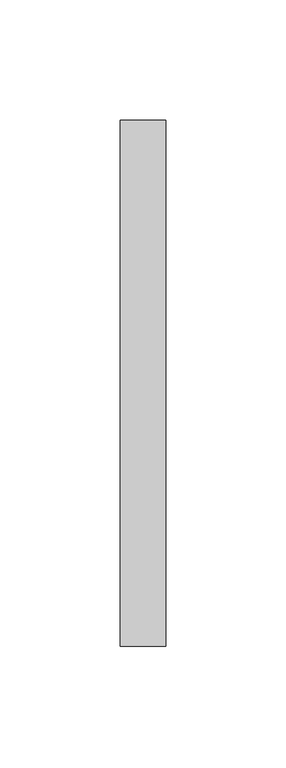
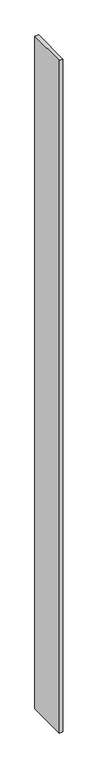
"""IFC4 building model written with IfcOpenShell, lengths in millimetres: proxy geometry, Inner panel1:Inner panel:306176:Inner panel:306176 : Inner panel1:Inner panel:306176:300391:Inner panel:306176:Inner panel:306176 : Inner panel1:Inner panel:306176:300391 : Inner panel1:Inner panel:306176:Inner panel:306176 : Inner panel1:Inner panel:306176:300391:2 : Inner panel1:Inner panel:306176:Inner panel:306176 : Inner panel1:Inner panel:306176:300391:Inner panel:306176:Inner panel:306176 : Inner panel1:Inner panel:306176:300391 : Inner panel1:Inner panel:306176:Inner panel:306176 : Inner panel1:Inner panel:306176:300391:300168."""

from ifc_helpers import new_model, si_unit, frame, origin, place, context, project, spatial, polyline, outline, extrude, source, transform, mapped, element, save


def generic_models_e7d118f8(model_context):
    return source(origin(), model_context, "Body", "SweptSolid", [
        extrude(outline(polyline([(570452.6367239, -578997.5163841), (570433.5867239, -578997.5163841), (570433.5867239, -578778.4413841), (570452.6367239, -578778.4413841), (570452.6367239, -578997.5163841)])), frame((0.0, 0.0, 25.4), z_axis=(0.0, 0.0, 1.0), x_axis=(1.0, 0.0, 0.0)), (0.0, 0.0, 1.0), 3689.35),
    ])


if __name__ == "__main__":
    model = new_model("IFC4")
    model_context = context("Model", 3, world=origin())
    ifc_project = project(units=[si_unit("LENGTHUNIT", "METRE", prefix="MILLI")], contexts=[model_context])
    site = spatial("IfcSite", under=ifc_project)
    building = spatial("IfcBuilding", under=site)
    placement = place(None, origin())
    generic_models_shape = generic_models_e7d118f8(model_context)
    element("IfcBuildingElementProxy", 1, Name="Inner panel1:Inner panel:306176:Inner panel:306176 : Inner panel1:Inner panel:306176:300391:Inner panel:306176:Inner panel:306176 : Inner panel1:Inner panel:306176:300391 : Inner panel1:Inner panel:306176:Inner panel:306176 : Inner panel1:Inner panel:306176:300391:2 : Inner panel1:Inner panel:306176:Inner panel:306176 : Inner panel1:Inner panel:306176:300391:Inner panel:306176:Inner panel:306176 : Inner panel1:Inner panel:306176:300391 : Inner panel1:Inner panel:306176:Inner panel:306176 : Inner panel1:Inner panel:306176:300391:300168", ObjectType="Inner panel1:Inner panel:306176:Inner panel:306176 : Inner panel1:Inner panel:306176:300391:Inner panel:306176:Inner panel:306176 : Inner panel1:Inner panel:306176:300391 : Inner panel1:Inner panel:306176:Inner panel:306176 : Inner panel1:Inner panel:306176:300391:2 : Inner panel1:Inner panel:306176:Inner panel:306176 : Inner panel1:Inner panel:306176:300391:Inner panel:306176:Inner panel:306176 : Inner panel1:Inner panel:306176:300391 : Inner panel1:Inner panel:306176:Inner panel:306176 : Inner panel1:Inner panel:306176:300391:300168", at=placement, inside=building, context=model_context, shape_type="MappedRepresentation", body=[
        mapped(generic_models_shape, transform((0.0, 0.0, 0.0), x_axis=(1.0, 0.0, 0.0), y_axis=(0.0, 1.0, 0.0), z_axis=(0.0, 0.0, 1.0))),
    ])
    save(model, "model.ifc")

# Revit data of these elements
# Type "Inner panel1:Inner panel:306176:Inner panel:306176 : Inner panel1:Inner panel:306176:300391:Inner panel:306176:Inner panel:306176 : Inner panel1:Inner panel:306176:300391 : Inner panel1:Inner panel:306176:Inner panel:306176 : Inner panel1:Inner panel:306176:300391:2 : Inner panel1:Inner panel:306176:Inner panel:306176 : Inner panel1:Inner panel:306176:300391:Inner panel:306176:Inner panel:306176 : Inner panel1:Inner panel:306176:300391 : Inner panel1:Inner panel:306176:Inner panel:306176 : Inner panel1:Inner panel:306176:300391:300168"
#   NameOverride = "Inner panel1:Inner panel:306176:Inner panel:306176 : Inner panel1:Inner panel:306176:300391:Inner panel:306176:Inner panel:306176 : Inner panel1:Inner panel:306176:300391 : Inner panel1:Inner panel:306176:Inner panel:306176 : Inner panel1:Inner panel:306176:300391:300168"
#   ObjectTypeOverride = "Inner panel:306176:Inner panel:306176 : Inner panel1:Inner panel:306176:300391 : Inner panel1:Inner panel:306176:Inner panel:306176 : Inner panel1:Inner panel:306176:300391"
#   Reference = "Inner panel"
#   Tag = "300168"
# Element 1 (IfcBuildingElementProxy, "Inner panel1:Inner panel:306176:Inner panel:306176 : Inner panel1:Inner panel:306176:300391:Inner panel:306176:Inner panel:306176 : Inner panel1:Inner panel:306176:300391 : Inner panel1:Inner panel:306176:Inner panel:306176 : Inner panel1:Inner panel:306176:300391:2 : Inner panel1:Inner panel:306176:Inner panel:306176 : Inner panel1:Inner panel:306176:300391:Inner panel:306176:Inner panel:306176 : Inner panel1:Inner panel:306176:300391 : Inner panel1:Inner panel:306176:Inner panel:306176 : Inner panel1:Inner panel:306176:300391:300168")
#   Materials on its faces: "¾” (CLASS A) FIRE RETARDANT PLYWOOD ...OR… IF 1/4\" GYP. BD UNDER PLYWOOD, FLAME SPREAD TO BE CLASS C -  (FINISH: GRADE B - PREFINISHED STAINED/SEALED) - 1/4\" GAP BTWN PANELS (FASTENERS T.B.D.)"
# Materials
#   "¾” (CLASS A) FIRE RETARDANT PLYWOOD ...OR… IF 1/4\" GYP. BD UNDER PLYWOOD, FLAME SPREAD TO BE CLASS C -  (FINISH: GRADE B - PREFINISHED STAINED/SEALED) - 1/4\" GAP BTWN PANELS (FASTENERS T.B.D.)": class "Wood", colour RGB 149 120 74, transparency 0, Description = "Plywood, sheathing grade", Cost = 0
